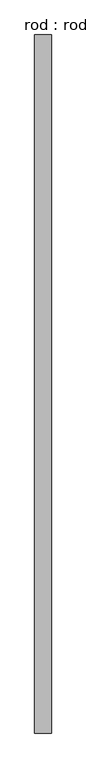
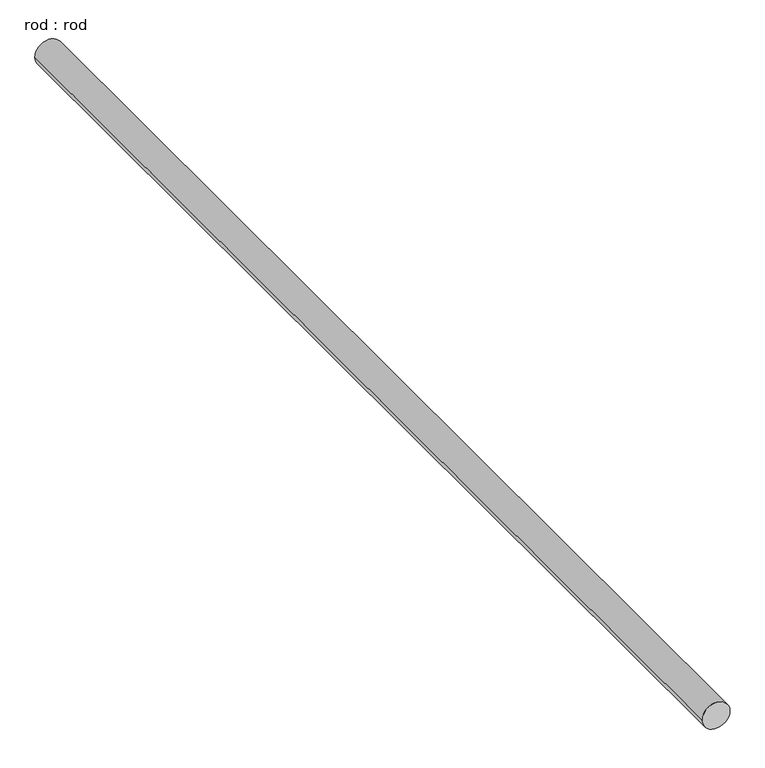
"""IFC4 building model written with IfcOpenShell, lengths in millimetres: proxy geometry, rod : rod."""

from ifc_helpers import new_model, si_unit, point, frame, frame_2d, origin, place, context, project, spatial, circle_curve, trimmed, segment, composite_curve, outline, extrude, source, transform, mapped, element, save


def rod_rod_2f919195(model_context):
    return source(origin(), model_context, "Body", "SweptSolid", [
        extrude(outline(composite_curve([segment(trimmed(circle_curve(frame_2d((0.0108462, 0.0)), 200.0), [point((0.0108462, 200.0))], [point((0.0108462, -200.0))], False, "CARTESIAN"), True, "CONTINUOUS"), segment(trimmed(circle_curve(frame_2d((0.0108462, 0.0)), 200.0), [point((0.0108462, -200.0))], [point((0.0108462, 200.0))], False, "CARTESIAN"), True, "CONTINUOUS")], self_intersect=False)), frame((0.0, -4282.2713847, 0.0), z_axis=(0.0, 1.0, 0.0), x_axis=(0.0, 0.0, 1.0)), (0.0, 0.0, 1.0), 16750.0),
    ])


if __name__ == "__main__":
    model = new_model("IFC4")
    model_context = context("Model", 3, world=origin())
    ifc_project = project(units=[si_unit("LENGTHUNIT", "METRE", prefix="MILLI")], contexts=[model_context])
    site = spatial("IfcSite", under=ifc_project)
    building = spatial("IfcBuilding", under=site)
    placement = place(None, origin())
    rod_rod_shape = rod_rod_2f919195(model_context)
    element("IfcBuildingElementProxy", 1, Name="rod : rod", ObjectType="rod : rod", at=placement, inside=building, context=model_context, shape_type="MappedRepresentation", body=[
        mapped(rod_rod_shape, transform((0.0, 0.0, 0.0), x_axis=(1.0, 0.0, 0.0), y_axis=(0.0, 1.0, 0.0), z_axis=(0.0, 0.0, 1.0))),
    ])
    save(model, "model.ifc")

# Revit data of these elements
# Type "rod : rod"
#   Default Elevation = 0
